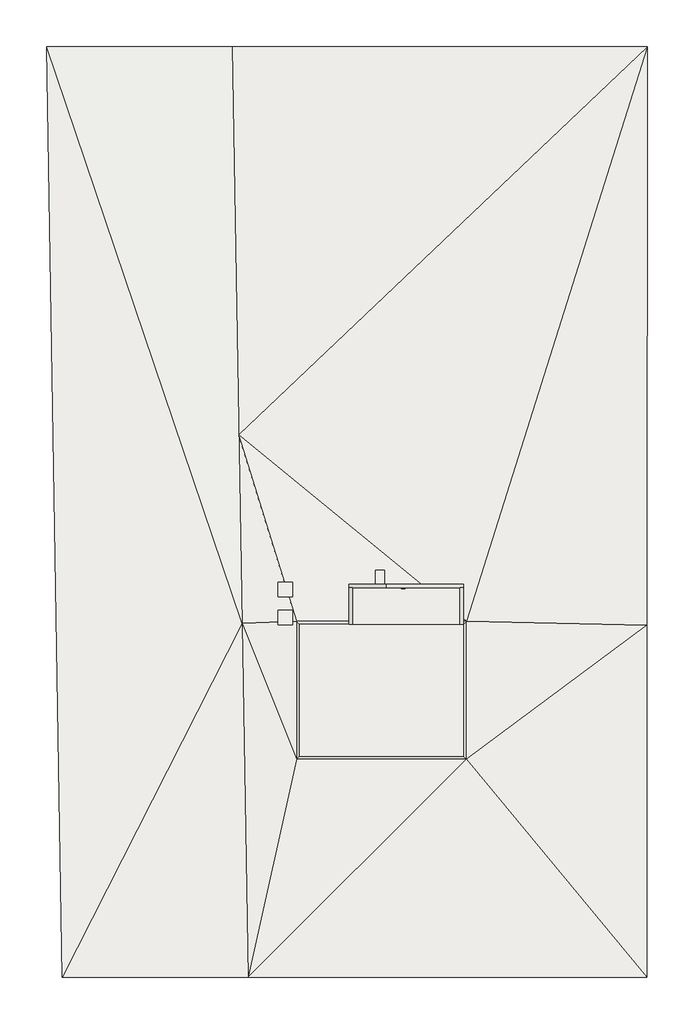
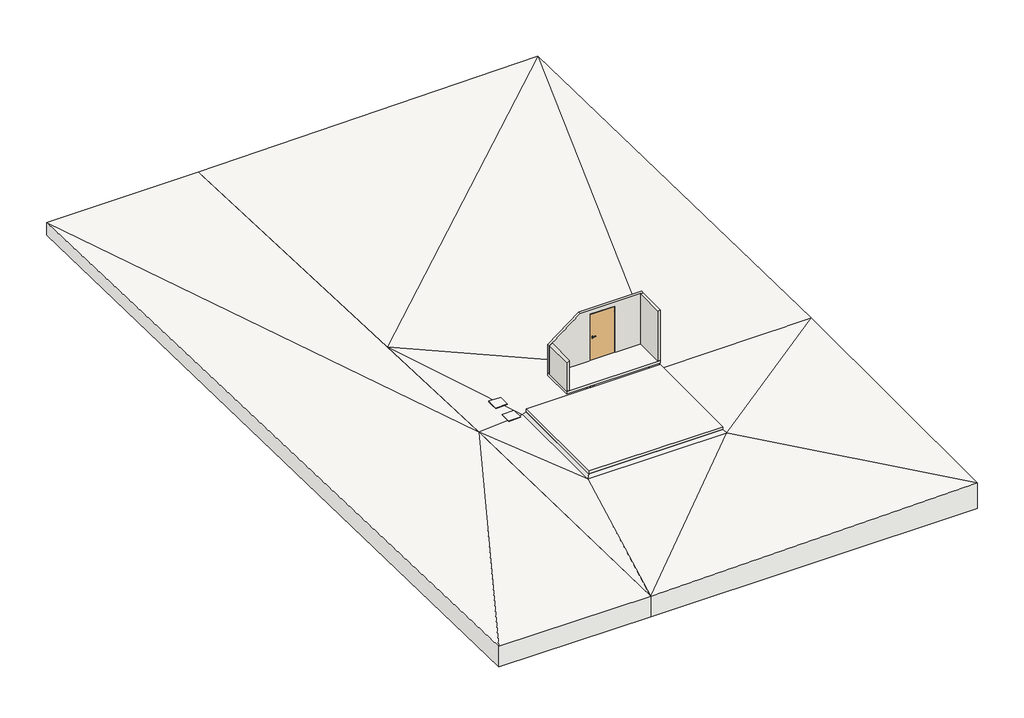
# Not in any storey: 7 slabs, 3 walls, 1 beam, 1 door.
"""IFC4 building model written with IfcOpenShell, lengths in millimetres."""

import ifcopenshell
import ifcopenshell.guid

model = None  # the IFC model being written
_history = None  # IfcOwnerHistory: only IFC2X3 demands one
_inside = {}  # id of a spatial element -> (the spatial element, [elements in it])
_under = {}  # id of a project, library or spatial element -> (it, [spatial elements below it])
_declared = {}  # id of a project -> (the project, [libraries it declares])
_typed = {}  # id of a type object -> (the type object, [elements of that type])
_made_of = {}  # id of a material, layer set ... -> (it, [elements and type objects made of it])


def new_model(schema):
    """Start an empty IFC model of exactly this schema.

    Asked for "IFC4X3", IfcOpenShell would pick the latest addendum, in which some entities
    have other attributes; the version numbers below select the first issue.
    IFC2X3 requires an IfcOwnerHistory on every rooted entity: one is made here for all.
    """
    global model, _history
    if schema == "IFC4X3":
        model = ifcopenshell.file(schema_version=(4, 3, 0, 0))
    else:
        model = ifcopenshell.file(schema=schema)
    _inside.clear()
    _under.clear()
    _declared.clear()
    _typed.clear()
    _made_of.clear()
    _history = None
    if model.schema == "IFC2X3":
        org = make("IfcOrganization", Name="unknown")
        user = make(
            "IfcPersonAndOrganization",
            ThePerson=make("IfcPerson", FamilyName="unknown"),
            TheOrganization=org,
        )
        app = make(
            "IfcApplication",
            ApplicationDeveloper=org,
            Version="unknown",
            ApplicationFullName="unknown",
            ApplicationIdentifier="unknown",
        )
        _history = make(
            "IfcOwnerHistory",
            OwningUser=user,
            OwningApplication=app,
            ChangeAction="ADDED",
            CreationDate=0,
        )
    return model


def make(cls, **values):
    """One entity of the class cls with the attributes given. An attribute that is None is left unset."""
    return model.create_entity(
        cls, **{name: value for name, value in values.items() if value is not None}
    )


def rooted(cls, **values):
    """An entity with a GlobalId (a new one), such as an element, a storey or a relation."""
    return make(cls, GlobalId=ifcopenshell.guid.new(), OwnerHistory=_history, **values)


def si_unit(unit_type, name, prefix=None):
    """IfcSIUnit, for example si_unit("LENGTHUNIT", "METRE", prefix="MILLI")."""
    return make("IfcSIUnit", UnitType=unit_type, Prefix=prefix, Name=name)


def assignment(units):
    """IfcUnitAssignment: the units of a project."""
    return None if units is None else make("IfcUnitAssignment", Units=units)


def point(xyz):
    """IfcCartesianPoint."""
    return None if xyz is None else make("IfcCartesianPoint", Coordinates=xyz)


def direction(xyz):
    """IfcDirection."""
    return None if xyz is None else make("IfcDirection", DirectionRatios=xyz)


def frame(location, z_axis=None, x_axis=None):
    """IfcAxis2Placement3D, a coordinate frame: its origin and axes. An axis left out is left unset."""
    return make(
        "IfcAxis2Placement3D",
        Location=point(location),
        Axis=direction(z_axis),
        RefDirection=direction(x_axis),
    )


def frame_2d(location, x_axis=None):
    """IfcAxis2Placement2D, a coordinate frame in the plane: its origin and x axis."""
    return make(
        "IfcAxis2Placement2D", Location=point(location), RefDirection=direction(x_axis)
    )


def origin():
    """The frame at (0, 0, 0) with its axes left unset."""
    return frame((0.0, 0.0, 0.0))


def place(relative_to, where):
    """IfcLocalPlacement: puts the frame where relative to a parent placement (None: the world)."""
    return make(
        "IfcLocalPlacement", PlacementRelTo=relative_to, RelativePlacement=where
    )


def context(
    kind, dimensions, precision=None, world=None, true_north=None, identifier=None
):
    """IfcGeometricRepresentationContext, for example the 3D "Model" context."""
    return make(
        "IfcGeometricRepresentationContext",
        ContextIdentifier=identifier,
        ContextType=kind,
        CoordinateSpaceDimension=dimensions,
        Precision=precision,
        WorldCoordinateSystem=world,
        TrueNorth=true_north,
    )


def project(units=None, contexts=None):
    """IfcProject with its units and contexts."""
    return rooted(
        "IfcProject",
        Name="project",
        RepresentationContexts=contexts,
        UnitsInContext=assignment(units),
    )


def spatial(cls, under=None, at=None, **own):
    """A site, building, storey or space (cls), placed at a placement, below another one or the project."""
    s = rooted(cls, ObjectPlacement=at, **own)
    if under is not None:
        _under.setdefault(under.id(), (under, []))[1].append(s)
    return s


def polyline(points):
    """IfcPolyline through the points."""
    return make("IfcPolyline", Points=[point(p) for p in points])


def circle_curve(where, radius):
    """IfcCircle in the frame where."""
    return make("IfcCircle", Position=where, Radius=radius)


def ellipse_curve(where, semi_axis1, semi_axis2):
    """IfcEllipse in the frame where."""
    return make(
        "IfcEllipse", Position=where, SemiAxis1=semi_axis1, SemiAxis2=semi_axis2
    )


def trimmed(basis, trim1, trim2, sense, master):
    """IfcTrimmedCurve: the piece of a basis curve between two trims."""
    return make(
        "IfcTrimmedCurve",
        BasisCurve=basis,
        Trim1=trim1,
        Trim2=trim2,
        SenseAgreement=sense,
        MasterRepresentation=master,
    )


def segment(curve, same_sense, transition):
    """IfcCompositeCurveSegment."""
    return make(
        "IfcCompositeCurveSegment",
        Transition=transition,
        SameSense=same_sense,
        ParentCurve=curve,
    )


def composite_curve(segments, self_intersect=None):
    """IfcCompositeCurve: segments joined end to end."""
    return make("IfcCompositeCurve", Segments=segments, SelfIntersect=self_intersect)


def outline(outer, holes=None, kind="AREA"):
    """IfcArbitraryClosedProfileDef: a profile drawn as a closed curve; with holes, ...WithVoids."""
    if holes is None:
        return make("IfcArbitraryClosedProfileDef", ProfileType=kind, OuterCurve=outer)
    return make(
        "IfcArbitraryProfileDefWithVoids",
        ProfileType=kind,
        OuterCurve=outer,
        InnerCurves=holes,
    )


def extrude(swept, where, along, depth):
    """IfcExtrudedAreaSolid: the profile swept, set in the frame where, extruded along a direction by depth."""
    return make(
        "IfcExtrudedAreaSolid",
        SweptArea=swept,
        Position=where,
        ExtrudedDirection=direction(along),
        Depth=depth,
    )


def faces_of(points, faces, orient=None, outer=None):
    """IfcFace entities. A face is a list of loops; a loop is a list of indices into points, from 0.

    orient and outer hold one flag for each loop. By default every Orientation is true, the
    first loop of a face is its IfcFaceOuterBound and the others are IfcFaceBound.
    """
    made = []
    for i, loops in enumerate(faces):
        bounds = []
        for j, loop in enumerate(loops):
            is_outer = j == 0 if outer is None else outer[i][j]
            bounds.append(
                make(
                    "IfcFaceOuterBound" if is_outer else "IfcFaceBound",
                    Bound=make("IfcPolyLoop", Polygon=[points[k] for k in loop]),
                    Orientation=True if orient is None else orient[i][j],
                )
            )
        made.append(make("IfcFace", Bounds=bounds))
    return made


def faceted_brep(points, faces, orient=None, outer=None, voids=None):
    """IfcFacetedBrep: a solid bounded by flat faces; with voids (closed shells), ...WithVoids."""
    shared = [point(p) for p in points]
    hull = make("IfcClosedShell", CfsFaces=faces_of(shared, faces, orient, outer))
    if voids is None:
        return make("IfcFacetedBrep", Outer=hull)
    return make(
        "IfcFacetedBrepWithVoids",
        Outer=hull,
        Voids=[
            make(cls, CfsFaces=faces_of(shared, fs, o, b)) for cls, fs, o, b in voids
        ],
    )


def shape(context_of_items, identifier, shape_type, items):
    """IfcShapeRepresentation: the items that make up one representation, for example the "Body"."""
    return make(
        "IfcShapeRepresentation",
        ContextOfItems=context_of_items,
        RepresentationIdentifier=identifier,
        RepresentationType=shape_type,
        Items=items,
    )


def source(mapping_origin, context_of_items, identifier, shape_type, items):
    """IfcRepresentationMap: a shape defined once, which mapped items show again and again."""
    return make(
        "IfcRepresentationMap",
        MappingOrigin=mapping_origin,
        MappedRepresentation=shape(context_of_items, identifier, shape_type, items),
    )


def transform(
    local_origin,
    x_axis=None,
    y_axis=None,
    z_axis=None,
    scale=None,
    scale2=None,
    scale3=None,
    uniform=True,
):
    """IfcCartesianTransformationOperator3D, or its non-uniform kind. x_axis, y_axis, z_axis: its Axis1, 2, 3."""
    if uniform:
        return make(
            "IfcCartesianTransformationOperator3D",
            Axis1=direction(x_axis),
            Axis2=direction(y_axis),
            LocalOrigin=point(local_origin),
            Scale=scale,
            Axis3=direction(z_axis),
        )
    return make(
        "IfcCartesianTransformationOperator3DnonUniform",
        Axis1=direction(x_axis),
        Axis2=direction(y_axis),
        LocalOrigin=point(local_origin),
        Scale=scale,
        Axis3=direction(z_axis),
        Scale2=scale2,
        Scale3=scale3,
    )


def mapped(mapping_source, mapping_target):
    """IfcMappedItem: shows the shape of a source again, moved by a transform."""
    return make(
        "IfcMappedItem", MappingSource=mapping_source, MappingTarget=mapping_target
    )


def made_of(thing, what):
    """Note that an element or type object is made of a material, layer set ...; save() writes the relation."""
    if what is not None:
        _made_of.setdefault(what.id(), (what, []))[1].append(thing)
    return thing


def element(
    cls,
    number,
    at=None,
    inside=None,
    cuts=None,
    type_object=None,
    material=None,
    context=None,
    identifier="Body",
    shape_type=None,
    held_by="IfcProductDefinitionShape",
    body=None,
    shapes=None,
    **own,
):
    """One element of the class cls, such as IfcWall. Its Tag is "e" and its number.

    at: its placement. inside: the storey or other place that contains it. cuts: it is an
    opening in that element (IfcRelVoidsElement). A single representation is given by context,
    identifier, shape_type and body (its items); several are given by shapes. held_by: the class
    of the entity that holds the representations. save() writes the other relations.
    """
    e = rooted(cls, Tag="e%d" % number, ObjectPlacement=at, **own)
    if body is not None:
        shapes = [shape(context, identifier, shape_type, body)]
    if shapes is not None:
        e.Representation = make(held_by, Representations=shapes)
    if inside is not None:
        _inside.setdefault(inside.id(), (inside, []))[1].append(e)
    if cuts is not None:
        rooted(
            "IfcRelVoidsElement", RelatingBuildingElement=cuts, RelatedOpeningElement=e
        )
    if type_object is not None:
        _typed.setdefault(type_object.id(), (type_object, []))[1].append(e)
    return made_of(e, material)


def aggregate(whole, parts):
    """IfcRelAggregates: a whole, such as a stair, and the parts it consists of."""
    return rooted("IfcRelAggregates", RelatingObject=whole, RelatedObjects=parts)


def save(model, path):
    """Write the relations noted so far, then the file.

    IfcRelAggregates (storeys below a building ...), IfcRelContainedInSpatialStructure (elements
    in a storey), IfcRelDefinesByType, IfcRelAssociatesMaterial and IfcRelDeclares: one each for
    every whole, place, type object, material and project.
    """
    for whole, parts in _under.values():
        aggregate(whole, parts)
    for where, things in _inside.values():
        rooted(
            "IfcRelContainedInSpatialStructure",
            RelatedElements=things,
            RelatingStructure=where,
        )
    for kind, things in _typed.values():
        rooted("IfcRelDefinesByType", RelatedObjects=things, RelatingType=kind)
    for what, things in _made_of.values():
        rooted("IfcRelAssociatesMaterial", RelatedObjects=things, RelatingMaterial=what)
    for by, libraries in _declared.values():
        rooted("IfcRelDeclares", RelatingContext=by, RelatedDefinitions=libraries)
    model.write(path)


def plane_surface(at):
    """IfcPlane: the flat surface through the origin of the frame at, square to its z axis."""
    return make("IfcPlane", Position=at)


def cylinder_surface(at, radius):
    """IfcCylindricalSurface: all points at the distance radius from the z axis of the frame at."""
    return make("IfcCylindricalSurface", Position=at, Radius=radius)


def advanced_brep(points, edges, surfaces, faces):
    """IfcAdvancedBrep: a solid bounded by faces that lie on surfaces and meet in shared edges.

    An edge is (start, end): straight between two places in points (the first is 0);
    or (start, end, curve); or (start, end, curve, False) where it runs against its curve.
    A face is (place in surfaces, loops), or (place, loops, False) where it looks against
    its surface's normal. A loop lists edges by number (the first is 1), with a minus sign
    where the edge is run from its end to its start. The first loop is the outer one.
    """
    corners = [point(p) for p in points]
    vertices = [make("IfcVertexPoint", VertexGeometry=c) for c in corners]
    made = []
    for start, end, *more in edges:
        made.append(
            make(
                "IfcEdgeCurve",
                EdgeStart=vertices[start],
                EdgeEnd=vertices[end],
                EdgeGeometry=more[0] if more else make("IfcPolyline", Points=[corners[start], corners[end]]),
                SameSense=more[1] if len(more) > 1 else True,
            )
        )
    hull = []
    for where, loops, *sense in faces:
        bounds = []
        for j, loop in enumerate(loops):
            ring = [make("IfcOrientedEdge", EdgeElement=made[abs(k) - 1], Orientation=k > 0) for k in loop]
            bounds.append(
                make(
                    "IfcFaceOuterBound" if j == 0 else "IfcFaceBound",
                    Bound=make("IfcEdgeLoop", EdgeList=ring),
                    Orientation=True,
                )
            )
        hull.append(make("IfcAdvancedFace", Bounds=bounds, FaceSurface=surfaces[where], SameSense=sense[0] if sense else True))
    return make("IfcAdvancedBrep", Outer=make("IfcClosedShell", CfsFaces=hull))


def holz_90_x_100_50d95c69(model_context):
    return source(origin(), model_context, "Body", "SweptSolid", [
        extrude(outline(polyline([(-638.5, -45.0), (-638.5, 45.0), (638.5, 45.0), (638.5, -45.0), (-638.5, -45.0)])), frame((0.0, 0.0, -50.0), z_axis=(0.0, 0.0, 1.0), x_axis=(1.0, 0.0, 0.0)), (0.0, 0.0, 1.0), 100.0),
    ])


def ml_1080_x_2101_9ecaf8c8(model_context):
    return source(origin(), model_context, "Body", "SolidModel", [
        faceted_brep([(515.0, -44.5, 0.0), (-515.0, -44.5, 0.0), (-515.0, -27.5, 0.0), (-500.0, -27.5, 0.0), (-500.0, 0.5, 0.0), (500.0, 0.5, 0.0), (500.0, -27.5, 0.0), (515.0, -27.5, 0.0), (515.0, -44.5, 2075.0), (-515.0, -44.5, 2075.0), (-515.0, -27.5, 2075.0), (-500.0, -27.5, 2060.0), (515.0, -27.5, 2075.0), (500.0, -27.5, 2060.0), (-500.0, 0.5, 2060.0), (500.0, 0.5, 2060.0)], [[[0, 1, 2, 3, 4, 5, 6, 7]], [[8, 9, 1, 0]], [[1, 9, 10, 2]], [[11, 3, 2, 10, 12, 7, 6, 13]], [[3, 11, 14, 4]], [[5, 4, 14, 15]], [[13, 6, 5, 15]], [[8, 0, 7, 12]], [[9, 8, 12, 10]], [[11, 13, 15, 14]]]),
        extrude(outline(composite_curve([segment(trimmed(circle_curve(frame_2d((527.0, -37.5)), 10.0), [point((517.0, -37.5))], [point((537.0, -37.5))], False, "CARTESIAN"), True, "CONTINUOUS"), segment(trimmed(circle_curve(frame_2d((527.0, -37.5)), 10.0), [point((537.0, -37.5))], [point((517.0, -37.5))], False, "CARTESIAN"), True, "CONTINUOUS")], self_intersect=False)), frame((0.0, 0.0, 1844.0), z_axis=(0.0, 0.0, 1.0), x_axis=(1.0, 0.0, 0.0)), (0.0, 0.0, 1.0), 25.0),
        extrude(outline(composite_curve([segment(trimmed(circle_curve(frame_2d((527.0, -37.5)), 10.0), [point((527.0, -27.5))], [point((518.339746, -32.5))], False, "CARTESIAN"), True, "CONTINUOUS"), segment(polyline([(518.339746, -32.5), (515.0, -32.5), (515.0, -27.5), (527.0, -27.5)]), True, "CONTINUOUS")], self_intersect=False)), frame((0.0, 0.0, 1794.0), z_axis=(0.0, 0.0, 1.0), x_axis=(1.0, 0.0, 0.0)), (0.0, 0.0, 1.0), 50.0),
        extrude(outline(composite_curve([segment(trimmed(circle_curve(frame_2d((527.0, -37.5)), 10.0), [point((517.0, -37.5))], [point((537.0, -37.5))], False, "CARTESIAN"), True, "CONTINUOUS"), segment(trimmed(circle_curve(frame_2d((527.0, -37.5)), 10.0), [point((537.0, -37.5))], [point((517.0, -37.5))], False, "CARTESIAN"), True, "CONTINUOUS")], self_intersect=False)), frame((0.0, 0.0, 1769.0), z_axis=(0.0, 0.0, 1.0), x_axis=(1.0, 0.0, 0.0)), (0.0, 0.0, 1.0), 25.0),
        extrude(outline(composite_curve([segment(trimmed(circle_curve(frame_2d((527.0, -37.5)), 10.0), [point((517.0, -37.5))], [point((537.0, -37.5))], False, "CARTESIAN"), True, "CONTINUOUS"), segment(trimmed(circle_curve(frame_2d((527.0, -37.5)), 10.0), [point((537.0, -37.5))], [point((517.0, -37.5))], False, "CARTESIAN"), True, "CONTINUOUS")], self_intersect=False)), frame((0.0, 0.0, 266.0), z_axis=(0.0, 0.0, 1.0), x_axis=(1.0, 0.0, 0.0)), (0.0, 0.0, 1.0), 25.0),
        extrude(outline(composite_curve([segment(trimmed(circle_curve(frame_2d((527.0, -37.5)), 10.0), [point((527.0, -27.5))], [point((518.339746, -32.5))], False, "CARTESIAN"), True, "CONTINUOUS"), segment(polyline([(518.339746, -32.5), (515.0, -32.5), (515.0, -27.5), (527.0, -27.5)]), True, "CONTINUOUS")], self_intersect=False)), frame((0.0, 0.0, 216.0), z_axis=(0.0, 0.0, 1.0), x_axis=(1.0, 0.0, 0.0)), (0.0, 0.0, 1.0), 50.0),
        extrude(outline(composite_curve([segment(trimmed(circle_curve(frame_2d((527.0, -37.5)), 10.0), [point((517.0, -37.5))], [point((537.0, -37.5))], False, "CARTESIAN"), True, "CONTINUOUS"), segment(trimmed(circle_curve(frame_2d((527.0, -37.5)), 10.0), [point((537.0, -37.5))], [point((517.0, -37.5))], False, "CARTESIAN"), True, "CONTINUOUS")], self_intersect=False)), frame((0.0, 0.0, 191.0), z_axis=(0.0, 0.0, 1.0), x_axis=(1.0, 0.0, 0.0)), (0.0, 0.0, 1.0), 25.0),
        advanced_brep(
        [(-420.0, -54.5, 1050.0), (-440.0, -54.5, 1050.0), (-440.0, -104.5, 1050.0), (-420.0, -84.5, 1050.0), (-310.0, -84.5, 1050.0), (-310.0, -104.5, 1050.0)],
        [
            (0, 1, circle_curve(frame((-430.0, -54.5, 1050.0), z_axis=(0.0, 1.0, 0.0), x_axis=(-1.0, 0.0, 0.0)), 10.0)),
            (1, 0, circle_curve(frame((-430.0, -54.5, 1050.0), z_axis=(0.0, 1.0, 0.0), x_axis=(-1.0, 0.0, 0.0)), 10.0)),
            (1, 2),
            (2, 3, ellipse_curve(frame((-430.0, -94.5, 1050.0), z_axis=(-0.7071067811865531, 0.7071067811865419, 0.0), x_axis=(0.707106781186542, 0.707106781186553, 0.0)), 14.1421356, 10.0)),
            (3, 0),
            (3, 2, ellipse_curve(frame((-430.0, -94.5, 1050.0), z_axis=(-0.7071067811865531, 0.7071067811865419, 0.0), x_axis=(0.707106781186542, 0.707106781186553, 0.0)), 14.1421356, 10.0)),
            (4, 5, circle_curve(frame((-310.0, -94.5, 1050.0), z_axis=(1.0, 0.0, 0.0), x_axis=(0.0, -1.0, 0.0)), 10.0)),
            (5, 4, circle_curve(frame((-310.0, -94.5, 1050.0), z_axis=(1.0, 0.0, 0.0), x_axis=(0.0, -1.0, 0.0)), 10.0)),
            (2, 5),
            (4, 3),
        ],
        [
            plane_surface(frame((-430.0, -54.5, 1050.0), z_axis=(0.0, 1.0, 0.0), x_axis=(0.0, 0.0, 1.0))),
            cylinder_surface(frame((-430.0, -54.5, 1050.0), z_axis=(0.0, 1.0, 0.0), x_axis=(-1.0, 0.0, 0.0)), 10.0),
            plane_surface(frame((-310.0, -94.5, 1050.0), z_axis=(1.0, 0.0, 0.0), x_axis=(0.0, 0.0, 1.0))),
            cylinder_surface(frame((-430.0, -94.5, 1050.0), z_axis=(-1.0, 0.0, 0.0), x_axis=(0.0, -1.0, 0.0)), 10.0),
        ],
        [
            (0, [[1, 2]]),
            (1, [[3, 4, 5, -2]]),
            (1, [[-5, 6, -3, -1]]),
            (2, [[7, 8]]),
            (3, [[9, -7, 10, -4]]),
            (3, [[-10, -8, -9, -6]]),
        ],
    ),
        extrude(outline(composite_curve([segment(trimmed(circle_curve(frame_2d((990.0, -430.0)), 20.0), [point((990.0, -450.0))], [point((990.0, -410.0))], False, "CARTESIAN"), True, "CONTINUOUS"), segment(trimmed(circle_curve(frame_2d((990.0, -430.0)), 20.0), [point((990.0, -410.0))], [point((990.0, -450.0))], False, "CARTESIAN"), True, "CONTINUOUS")], self_intersect=False), holes=[composite_curve([segment(polyline([(976.4601385, -432.397268), (988.4749012, -432.397268)]), True, "CONTINUOUS"), segment(trimmed(circle_curve(frame_2d((995.0361633, -430.0)), 6.9854888), [point((988.4749012, -432.397268))], [point((988.4749012, -427.602732))], True, "CARTESIAN"), True, "CONTINUOUS"), segment(polyline([(988.4749012, -427.602732), (976.4601385, -427.602732)]), True, "CONTINUOUS"), segment(trimmed(circle_curve(frame_2d((976.4601385, -430.0)), 2.397268), [point((976.4601385, -427.602732))], [point((976.4601385, -432.397268))], True, "CARTESIAN"), True, "CONTINUOUS")], self_intersect=False)]), frame((0.0, -54.5, 0.0), z_axis=(0.0, 1.0, 0.0), x_axis=(0.0, 0.0, 1.0)), (0.0, 0.0, 1.0), 10.0),
        advanced_brep(
        [(-420.0, -54.5, 1050.0), (-440.0, -54.5, 1050.0), (-440.0, -104.5, 1050.0), (-420.0, -84.5, 1050.0), (-310.0, -84.5, 1050.0), (-310.0, -104.5, 1050.0)],
        [
            (0, 1, circle_curve(frame((-430.0, -54.5, 1050.0), z_axis=(0.0, 1.0, 0.0), x_axis=(-1.0, 0.0, 0.0)), 10.0)),
            (1, 0, circle_curve(frame((-430.0, -54.5, 1050.0), z_axis=(0.0, 1.0, 0.0), x_axis=(-1.0, 0.0, 0.0)), 10.0)),
            (1, 2),
            (2, 3, ellipse_curve(frame((-430.0, -94.5, 1050.0), z_axis=(-0.7071067811865537, 0.7071067811865414, 0.0), x_axis=(0.7071067811865414, 0.7071067811865536, 0.0)), 14.1421356, 10.0)),
            (3, 0),
            (3, 2, ellipse_curve(frame((-430.0, -94.5, 1050.0), z_axis=(-0.7071067811865537, 0.7071067811865414, 0.0), x_axis=(0.7071067811865414, 0.7071067811865536, 0.0)), 14.1421356, 10.0)),
            (4, 5, circle_curve(frame((-310.0, -94.5, 1050.0), z_axis=(1.0, 0.0, 0.0), x_axis=(0.0, -1.0, 0.0)), 10.0)),
            (5, 4, circle_curve(frame((-310.0, -94.5, 1050.0), z_axis=(1.0, 0.0, 0.0), x_axis=(0.0, -1.0, 0.0)), 10.0)),
            (2, 5),
            (4, 3),
        ],
        [
            plane_surface(frame((-430.0, -54.5, 1050.0), z_axis=(0.0, 1.0, 0.0), x_axis=(0.0, 0.0, 1.0))),
            cylinder_surface(frame((-430.0, -54.5, 1050.0), z_axis=(0.0, 1.0, 0.0), x_axis=(-1.0, 0.0, 0.0)), 10.0),
            plane_surface(frame((-310.0, -94.5, 1050.0), z_axis=(1.0, 0.0, 0.0), x_axis=(0.0, 0.0, 1.0))),
            cylinder_surface(frame((-430.0, -94.5, 1050.0), z_axis=(-1.0, 0.0, 0.0), x_axis=(0.0, -1.0, 0.0)), 10.0),
        ],
        [
            (0, [[1, 2]]),
            (1, [[3, 4, 5, -2]]),
            (1, [[-5, 6, -3, -1]]),
            (2, [[7, 8]]),
            (3, [[9, -7, 10, -4]]),
            (3, [[-10, -8, -9, -6]]),
        ],
    ),
        extrude(outline(composite_curve([segment(trimmed(circle_curve(frame_2d((1050.0, -430.0)), 20.0), [point((1050.0, -450.0))], [point((1050.0, -410.0))], False, "CARTESIAN"), True, "CONTINUOUS"), segment(trimmed(circle_curve(frame_2d((1050.0, -430.0)), 20.0), [point((1050.0, -410.0))], [point((1050.0, -450.0))], False, "CARTESIAN"), True, "CONTINUOUS")], self_intersect=False)), frame((0.0, -54.5, 0.0), z_axis=(0.0, 1.0, 0.0), x_axis=(0.0, 0.0, 1.0)), (0.0, 0.0, 1.0), 10.0),
        advanced_brep(
        [(-420.0, 10.5, 1050.0), (-440.0, 10.5, 1050.0), (-420.0, 40.5, 1050.0), (-440.0, 60.5, 1050.0), (-310.0, 40.5, 1050.0), (-310.0, 60.5, 1050.0)],
        [
            (0, 1, circle_curve(frame((-430.0, 10.5, 1050.0), z_axis=(0.0, -1.0, 0.0), x_axis=(-1.0, 0.0, 0.0)), 10.0)),
            (1, 0, circle_curve(frame((-430.0, 10.5, 1050.0), z_axis=(0.0, -1.0, 0.0), x_axis=(-1.0, 0.0, 0.0)), 10.0)),
            (0, 2),
            (2, 3, ellipse_curve(frame((-430.0, 50.5, 1050.0), z_axis=(-0.7071067811865486, -0.7071067811865464, 0.0), x_axis=(0.7071067811865464, -0.7071067811865488, 0.0)), 14.1421356, 10.0)),
            (3, 1),
            (3, 2, ellipse_curve(frame((-430.0, 50.5, 1050.0), z_axis=(-0.7071067811865486, -0.7071067811865464, 0.0), x_axis=(0.7071067811865464, -0.7071067811865488, 0.0)), 14.1421356, 10.0)),
            (4, 5, circle_curve(frame((-310.0, 50.5, 1050.0), z_axis=(1.0, 0.0, 0.0), x_axis=(0.0, 1.0, 0.0)), 10.0)),
            (5, 4, circle_curve(frame((-310.0, 50.5, 1050.0), z_axis=(1.0, 0.0, 0.0), x_axis=(0.0, 1.0, 0.0)), 10.0)),
            (2, 4),
            (5, 3),
        ],
        [
            plane_surface(frame((-430.0, 10.5, 1050.0), z_axis=(0.0, -1.0, 0.0), x_axis=(0.0, 0.0, 1.0))),
            cylinder_surface(frame((-430.0, 10.5, 1050.0), z_axis=(0.0, -1.0, 0.0), x_axis=(-1.0, 0.0, 0.0)), 10.0),
            plane_surface(frame((-310.0, 50.5, 1050.0), z_axis=(1.0, 0.0, 0.0), x_axis=(0.0, 0.0, 1.0))),
            cylinder_surface(frame((-430.0, 50.5, 1050.0), z_axis=(-1.0, 0.0, 0.0), x_axis=(0.0, 1.0, 0.0)), 10.0),
        ],
        [
            (0, [[1, 2]]),
            (1, [[-1, 3, 4, 5]]),
            (1, [[-2, -5, 6, -3]]),
            (2, [[7, 8]]),
            (3, [[-4, 9, -8, 10]]),
            (3, [[-6, -10, -7, -9]]),
        ],
    ),
        extrude(outline(composite_curve([segment(trimmed(circle_curve(frame_2d((990.0, -430.0)), 20.0), [point((990.0, -450.0))], [point((990.0, -410.0))], False, "CARTESIAN"), True, "CONTINUOUS"), segment(trimmed(circle_curve(frame_2d((990.0, -430.0)), 20.0), [point((990.0, -410.0))], [point((990.0, -450.0))], False, "CARTESIAN"), True, "CONTINUOUS")], self_intersect=False), holes=[composite_curve([segment(polyline([(976.4601385, -432.397268), (988.4749012, -432.397268)]), True, "CONTINUOUS"), segment(trimmed(circle_curve(frame_2d((995.0361633, -430.0)), 6.9854888), [point((988.4749012, -432.397268))], [point((988.4749012, -427.602732))], True, "CARTESIAN"), True, "CONTINUOUS"), segment(polyline([(988.4749012, -427.602732), (976.4601385, -427.602732)]), True, "CONTINUOUS"), segment(trimmed(circle_curve(frame_2d((976.4601385, -430.0)), 2.397268), [point((976.4601385, -427.602732))], [point((976.4601385, -432.397268))], True, "CARTESIAN"), True, "CONTINUOUS")], self_intersect=False)]), frame((0.0, 0.5, 0.0), z_axis=(0.0, 1.0, 0.0), x_axis=(0.0, 0.0, 1.0)), (0.0, 0.0, 1.0), 10.0),
        advanced_brep(
        [(-420.0, 10.5, 1050.0), (-440.0, 10.5, 1050.0), (-420.0, 40.5, 1050.0), (-440.0, 60.5, 1050.0), (-310.0, 40.5, 1050.0), (-310.0, 60.5, 1050.0)],
        [
            (0, 1, circle_curve(frame((-430.0, 10.5, 1050.0), z_axis=(0.0, -1.0, 0.0), x_axis=(-1.0, 0.0, 0.0)), 10.0)),
            (1, 0, circle_curve(frame((-430.0, 10.5, 1050.0), z_axis=(0.0, -1.0, 0.0), x_axis=(-1.0, 0.0, 0.0)), 10.0)),
            (0, 2),
            (2, 3, ellipse_curve(frame((-430.0, 50.5, 1050.0), z_axis=(-0.7071067811865491, -0.7071067811865459, 0.0), x_axis=(0.7071067811865458, -0.7071067811865492, 0.0)), 14.1421356, 10.0)),
            (3, 1),
            (3, 2, ellipse_curve(frame((-430.0, 50.5, 1050.0), z_axis=(-0.7071067811865491, -0.7071067811865459, 0.0), x_axis=(0.7071067811865458, -0.7071067811865492, 0.0)), 14.1421356, 10.0)),
            (4, 5, circle_curve(frame((-310.0, 50.5, 1050.0), z_axis=(1.0, 0.0, 0.0), x_axis=(0.0, 1.0, 0.0)), 10.0)),
            (5, 4, circle_curve(frame((-310.0, 50.5, 1050.0), z_axis=(1.0, 0.0, 0.0), x_axis=(0.0, 1.0, 0.0)), 10.0)),
            (2, 4),
            (5, 3),
        ],
        [
            plane_surface(frame((-430.0, 10.5, 1050.0), z_axis=(0.0, -1.0, 0.0), x_axis=(0.0, 0.0, 1.0))),
            cylinder_surface(frame((-430.0, 10.5, 1050.0), z_axis=(0.0, -1.0, 0.0), x_axis=(-1.0, 0.0, 0.0)), 10.0),
            plane_surface(frame((-310.0, 50.5, 1050.0), z_axis=(1.0, 0.0, 0.0), x_axis=(0.0, 0.0, 1.0))),
            cylinder_surface(frame((-430.0, 50.5, 1050.0), z_axis=(-1.0, 0.0, 0.0), x_axis=(0.0, 1.0, 0.0)), 10.0),
        ],
        [
            (0, [[1, 2]]),
            (1, [[-1, 3, 4, 5]]),
            (1, [[-2, -5, 6, -3]]),
            (2, [[7, 8]]),
            (3, [[-4, 9, -8, 10]]),
            (3, [[-6, -10, -7, -9]]),
        ],
    ),
        extrude(outline(composite_curve([segment(trimmed(circle_curve(frame_2d((1050.0, -430.0)), 20.0), [point((1050.0, -450.0))], [point((1050.0, -410.0))], False, "CARTESIAN"), True, "CONTINUOUS"), segment(trimmed(circle_curve(frame_2d((1050.0, -430.0)), 20.0), [point((1050.0, -410.0))], [point((1050.0, -450.0))], False, "CARTESIAN"), True, "CONTINUOUS")], self_intersect=False)), frame((0.0, 0.5, 0.0), z_axis=(0.0, 1.0, 0.0), x_axis=(0.0, 0.0, 1.0)), (0.0, 0.0, 1.0), 10.0),
        faceted_brep([(-500.0, -27.5, 0.0), (-540.0, -27.5, 0.0), (-540.0, 27.5, 0.0), (-485.0, 27.5, 0.0), (-485.0, 0.5, 0.0), (-500.0, 0.5, 0.0), (-500.0, 0.5, 2060.0), (-500.0, -27.5, 2060.0), (-485.0, 0.5, 2045.0), (485.0, 0.5, 2045.0), (485.0, 0.5, 0.0), (500.0, 0.5, 0.0), (500.0, 0.5, 2060.0), (-485.0, 27.5, 2045.0), (-540.0, 27.5, 2100.0), (540.0, 27.5, 2100.0), (540.0, 27.5, 0.0), (485.0, 27.5, 0.0), (485.0, 27.5, 2045.0), (-540.0, -27.5, 2100.0), (500.0, -27.5, 2060.0), (500.0, -27.5, 0.0), (540.0, -27.5, 0.0), (540.0, -27.5, 2100.0)], [[[0, 1, 2, 3, 4, 5]], [[5, 6, 7, 0]], [[4, 8, 9, 10, 11, 12, 6, 5]], [[3, 13, 8, 4]], [[2, 14, 15, 16, 17, 18, 13, 3]], [[1, 19, 14, 2]], [[0, 7, 20, 21, 22, 23, 19, 1]], [[23, 22, 16, 15]], [[21, 11, 10, 17, 16, 22]], [[12, 11, 21, 20]], [[18, 17, 10, 9]], [[19, 23, 15, 14]], [[13, 18, 9, 8]], [[6, 12, 20, 7]]]),
    ])


def einzelfundament_stb_500_x_500_x_300_3619195b(model_context):
    return source(origin(), model_context, "Body", "SweptSolid", [
        extrude(outline(polyline([(250.0, 250.0), (250.0, -250.0), (-250.0, -250.0), (-250.0, 250.0), (250.0, 250.0)])), frame((0.0, 0.0, -300.0), z_axis=(0.0, 0.0, 1.0), x_axis=(1.0, 0.0, 0.0)), (0.0, 0.0, 1.0), 300.0),
    ])


model = new_model("IFC4")

# Units and contexts
model_context = context("Model", 3, world=origin())
ifc_project = project(units=[si_unit("LENGTHUNIT", "METRE", prefix="MILLI")], contexts=[model_context])

# Site, building
site = spatial("IfcSite", under=ifc_project)
building = spatial("IfcBuilding", under=site)

# Beam
placement = place(None, origin())
holz_90_x_100_shape = holz_90_x_100_50d95c69(model_context)
element("IfcBeam", 1, ObjectType="Holz Träger - rechteckig : Holz 90 x 100", at=placement, inside=building, context=model_context, shape_type="MappedRepresentation", body=[
    mapped(holz_90_x_100_shape, transform((9139.843584, 9402.7803922, -270.0), x_axis=(0.0, -1.0, 0.0), y_axis=(1.0, 0.0, 0.0), z_axis=(0.0, 0.0, 1.0))),
])

# Door
ml_1080_x_2101_shape = ml_1080_x_2101_9ecaf8c8(model_context)
element("IfcDoor", 2, ObjectType="TU DF 1 - Pfostenstock Falztüre : ML - 1080 x 2101", at=placement, inside=building, context=model_context, shape_type="MappedRepresentation", body=[
    mapped(ml_1080_x_2101_shape, transform((10322.9226469, 10084.5272422, -100.0), x_axis=(1.0, 0.0, 0.0), y_axis=(0.0, 1.0, 0.0), z_axis=(0.0, 0.0, 1.0))),
])

# Slabs
element("IfcSlab", 3, ObjectType="WD 120 hart", at=placement, inside=building, context=model_context, shape_type="SweptSolid", body=[
    extrude(outline(polyline([(12052.9226469, 8754.5272422), (12052.9226469, 4144.5272422), (6332.9226469, 4144.5272422), (6332.9226469, 8754.5272422), (12052.9226469, 8754.5272422)])), frame((0.0, 0.0, -420.0), z_axis=(0.0, 0.0, 1.0), x_axis=(1.0, 0.0, 0.0)), (0.0, 0.0, 1.0), 120.0),
])
element("IfcSlab", 4, ObjectType="AL Grünfläche", at=placement, inside=building, context=model_context, shape_type="Brep", body=[
    faceted_brep([(18451.9869184, 28873.5069375, -1560.9044), (18448.9881934, 8708.0675618, -1560.9044), (18447.1199211, -3557.1970822, -1560.9044), (4539.8145475, -3555.0786825, -1560.9044), (4328.9058413, 8779.6808532, -1560.9044), (3985.3098426, 28871.3033595, -1560.9044), (18451.9869184, 28873.5069375, -838.5044), (18448.9881934, 8708.0675618, -398.9094998), (18447.1199211, -3557.1970822, -400.9044), (4539.8145475, -3555.0786825, -642.6582175), (4328.9058413, 8779.6808532, -645.3457), (4216.6527387, 15343.6249499, -761.8881193), (3985.3098426, 28871.3033595, -1002.0712139), (6232.9226469, 4044.5272422, -560.9044), (12152.9226469, 4044.5272422, -560.9044), (6332.9226469, 8754.5272422, -420.0), (6332.9226469, 4144.5272422, -420.0), (12052.9226469, 4144.5272422, -420.0), (12052.9226469, 8754.5272422, -420.0), (12152.9226469, 8854.5272422, -560.9044), (6232.9226469, 8854.5272422, -560.9044)], [[[0, 1, 2, 3, 4, 5]], [[1, 0, 6, 7]], [[2, 1, 7, 8]], [[3, 2, 8, 9]], [[4, 3, 9, 10]], [[5, 4, 10, 11, 12]], [[0, 5, 12, 6]], [[10, 9, 13]], [[9, 8, 14]], [[12, 11, 6]], [[8, 7, 14]], [[15, 16, 17, 18]], [[15, 18, 19, 20]], [[7, 19, 14]], [[9, 14, 13]], [[17, 14, 19, 18]], [[16, 13, 14, 17]], [[15, 20, 13, 16]], [[10, 20, 11]], [[10, 13, 20]], [[11, 20, 19]], [[11, 19, 6]], [[7, 6, 19]]]),
])
element("IfcSlab", 5, ObjectType="AL Asphalt", at=placement, inside=building, context=model_context, shape_type="Brep", body=[
    faceted_brep([(4328.9058413, 8779.6808532, -1560.9044), (4539.8145475, -3555.0786825, -1560.9044), (-1931.6832245, -3555.0786825, -1560.9044), (-2486.2197616, 28871.3033595, -1560.9044), (3985.3098426, 28871.3033595, -1560.9044), (4328.9058413, 8779.6808532, -645.3456973), (4539.8145475, -3555.0786825, -642.6582175), (-1931.6832245, -3555.0786825, -642.7044), (-2486.2197616, 28871.3033595, -1002.1044), (3985.3098426, 28871.3033595, -1002.0712139)], [[[0, 1, 2, 3, 4]], [[1, 0, 5, 6]], [[2, 1, 6, 7]], [[3, 2, 7, 8]], [[4, 3, 8, 9]], [[0, 4, 9, 5]], [[9, 8, 5]], [[8, 7, 5]], [[7, 6, 5]]]),
])
element("IfcSlab", 6, ObjectType="Einzelfundament : STB 1870 x 300 x 500", at=placement, inside=building, context=model_context, shape_type="SweptSolid", body=[
    extrude(outline(polyline([(8989.843584, 10634.0293422), (9289.843584, 10634.0293422), (9289.843584, 8764.0293422), (8989.843584, 8764.0293422), (8989.843584, 10634.0293422)])), frame((0.0, 0.0, -820.0), z_axis=(0.0, 0.0, 1.0), x_axis=(1.0, 0.0, 0.0)), (0.0, 0.0, 1.0), 500.0),
])
einzelfundament_stb_500_x_500_x_300_shape = einzelfundament_stb_500_x_500_x_300_3619195b(model_context)
element("IfcSlab", 7, ObjectType="Einzelfundament : STB 500 x 500 x 300", at=placement, inside=building, context=model_context, shape_type="MappedRepresentation", body=[
    mapped(einzelfundament_stb_500_x_500_x_300_shape, transform((5835.8451291, 8984.5272422, -560.9044), x_axis=(1.0, 0.0, 0.0), y_axis=(0.0, 1.0, 0.0), z_axis=(0.0, 0.0, 1.0))),
])
element("IfcSlab", 8, ObjectType="Einzelfundament : STB 500 x 500 x 300", at=placement, inside=building, context=model_context, shape_type="MappedRepresentation", body=[
    mapped(einzelfundament_stb_500_x_500_x_300_shape, transform((5835.8451291, 9958.5272422, -560.9044), x_axis=(1.0, 0.0, 0.0), y_axis=(0.0, 1.0, 0.0), z_axis=(0.0, 0.0, 1.0))),
])
element("IfcSlab", 9, ObjectType="KLH 120", at=placement, inside=building, context=model_context, shape_type="SweptSolid", body=[
    extrude(outline(polyline([(12052.9226469, 8754.5272422), (8052.9226469, 8754.5272422), (8052.9226469, 10144.5272422), (12052.9226469, 10144.5272422), (12052.9226469, 8754.5272422)])), frame((0.0, 0.0, -220.0), z_axis=(0.0, 0.0, 1.0), x_axis=(1.0, 0.0, 0.0)), (0.0, 0.0, 1.0), 120.0),
])

# Walls
element("IfcWall", 10, ObjectType="KLH 120", at=placement, inside=building, context=model_context, shape_type="Brep", body=[
    faceted_brep([(12052.9226469, 10144.5272422, 2170.0), (12052.9226469, 10144.5272422, -100.0), (10862.9226469, 10144.5272422, -100.0), (10862.9226469, 10144.5272422, 2000.0), (9782.9226469, 10144.5272422, 2000.0), (9782.9226469, 10144.5272422, -100.0), (8052.9226469, 10144.5272422, -100.0), (8052.9226469, 10144.5272422, 1165.8420612), (9374.1830316, 10144.5272422, 2170.0), (12052.9226469, 10024.5272422, -100.0), (12052.9226469, 10024.5272422, 2170.0), (11932.9226469, 10024.5272422, 2170.0), (9374.1830316, 10024.5272422, 2170.0), (8172.9226469, 10024.5272422, 1257.0420654), (8052.9226469, 10024.5272422, 1165.8420612), (8052.9226469, 10024.5272422, -100.0), (8172.9226469, 10024.5272422, -100.0), (9782.9226469, 10024.5272422, -100.0), (9782.9226469, 10024.5272422, 2000.0), (10862.9226469, 10024.5272422, 2000.0), (10862.9226469, 10024.5272422, -100.0), (11932.9226469, 10024.5272422, -100.0)], [[[0, 1, 2, 3, 4, 5, 6, 7, 8]], [[9, 10, 11, 12, 13, 14, 15, 16, 17, 18, 19, 20, 21]], [[1, 9, 21, 20, 2]], [[15, 6, 5, 17, 16]], [[19, 3, 2, 20]], [[4, 18, 17, 5]], [[3, 19, 18, 4]], [[1, 0, 10, 9]], [[7, 6, 15, 14]], [[10, 0, 8, 12, 11]], [[7, 14, 13, 12, 8]]]),
])
element("IfcWall", 11, ObjectType="KLH 120", at=placement, inside=building, context=model_context, shape_type="SweptSolid", body=[
    extrude(outline(polyline([(12052.9226469, 10024.5272422), (12052.9226469, 8754.5272422), (11932.9226469, 8754.5272422), (11932.9226469, 10024.5272422), (12052.9226469, 10024.5272422)])), frame((0.0, 0.0, -100.0), z_axis=(0.0, 0.0, 1.0), x_axis=(1.0, 0.0, 0.0)), (0.0, 0.0, 1.0), 2270.0),
])
element("IfcWall", 12, ObjectType="KLH 120", at=placement, inside=building, context=model_context, shape_type="SweptSolid", body=[
    extrude(outline(polyline([(-100.0, 8172.9226469), (1257.0420654, 8172.9226469), (1165.8420612, 8052.9226469), (-100.0, 8052.9226469), (-100.0, 8172.9226469)])), frame((0.0, 8754.5272422, 0.0), z_axis=(0.0, 1.0, 0.0), x_axis=(0.0, 0.0, 1.0)), (0.0, 0.0, 1.0), 1270.0),
])

save(model, "model.ifc")

# Revit data of these elements
# Type "Holz Träger - rechteckig : Holz 90 x 100"
#   Type Comments = "B/H=9/10cm"
#   Perimeter = 0.38 m²/m
#   Moment of Inertia strong axis = 750.00 cm⁴
#   Moment of Inertia weak axis = 607.50 cm⁴
#   Section Area = 90.0 cm²
#   Length [instance default] = 1.524 m
#   Height = 10.0 cm
#   Width = 9.0 cm
#   B = 0.090 m
#   H = 0.100 m
#   Structural Material = Holz - C 24 Cl.1
# Type "TU DF 1 - Pfostenstock Falztüre : ML - 1080 x 2101"
#   Type IfcGUID = "32vBIxahr8bQdQw1D1hUMo"
#   Type Mark = "235"
#   Operation = "SINGLE_SWING_RIGHT"
#   URL = "http://www.autodesk.de/BIM"
#   Type Comments = "Pfostenstock Falztüre"
#   Form Tür = "rechteckig"
#   Description = "1-teilig"
#   Ausführung Zarge = "Blockzarge"
#   Anzahl Seitenteile = "0"
#   Anzahl Oberlichter = "0"
#   Anzahl Flügel = "einflügelig"
#   Anschlag- / Bewegungsart Tür = "Drehflügeltür"
#   Analytic Construction = "<Keine Auswahl>"
#   Winkel Öffnungsbogen [instance default] = 90.00°
#   Wandstärke Gesamt [instance default] = 0.300 m
#   Wandstärke [instance default] = 0.300 m
#   Wandaufbau Gegenbandseite [instance default] = 0.000 m
#   Wandaufbau Bandseite [instance default] = 0.000 m
#   Rough Height [instance default] = 2.280 m
#   Rough Width = 1.080 m
#   Randabstand Öffnungssymbol = 0.000 m
#   Rahmentiefe = 0.055 m
#   Rahmendicke = 0.055 m
#   Höhe ab FBOK = 2.100 m
#   Fußbodenaufbau [instance default] = 0.180 m
#   Height [instance default] = 2.100 m
#   Falztiefe = 0.028 m
#   Falzaufschlag = 0.017 m
#   Einbautiefe [instance default] = 0.080 m
#   Durchgangshöhe = 2.045 m
#   Durchgangsbreite = 0.970 m
#   Drückerhöhe = 1.050 m
#   Thickness = 0.045 m
#   Width = 1.080 m
#   B_Einbautiefe [instance default] = 0.1225 m
#   Angabe Maueröffnungsmaß Höhe = 2.100 m
#   Angabe Maueröffnungsmaß Breite = 1.080 m
#   Angabe Lichter Durchgang Höhe = 2.000 m
#   Angabe Lichter Durchgang Breite = 0.800 m
#   Zylinderrosette [instance default] = yes
#   Tür mit Anschlag [instance default] = no
#   Pfostenstock Wandmittig eingebaut [instance default] = yes
#   Kollisionskörper einschalten [instance default] = no
#   Knauf Innenseite [instance default] = no
#   Knauf Außenseite [instance default] = no
#   Höhe ab FBOK berechnen = yes
#   Größenberechnung über Maueröffnungsmaß = yes
#   Größenberechnung über Lichten Durchgang = no
#   Grundrissdarstellung Türsturz [instance default] = no
#   Drücker Bandseite [instance default] = yes
#   Drücker Gegenbandseite [instance default] = yes
#   Türblatt [instance default] = none
#   Sichtbeschläge [instance default] = none
#   Rahmen vertikal [instance default] = none
#   Rahmen horizontal [instance default] = none
#   Kollisionskörper [instance default] = none
#   Function = (empty or 0)
#   Wall Closure = (empty or 0)
#   Fire Rating = ""
# Type "WD 120 hart"
#   Type IfcGUID = "0KFvTt6w11YhWph5GwwxlC"
#   Type Comments = ""
#   Description = "WD_120_hart"
#   Function = 1
#   Filter Tragend / Nichttragend = no
#   Layers, outside or top first: 0.120 m "Dämmung - hart" (function 4)
# Type "AL Grünfläche"
#   Type Comments = ""
#   Description = "AL Grünfläche"
#   Function = 0
#   Filter Tragend / Nichttragend = no
#   Layers, outside or top first: 1.000 m "Umgebung - Erde" (function 4)
# Type "AL Asphalt"
#   Type Comments = ""
#   Description = "AL Asphalt"
#   Function = 0
#   Filter Tragend / Nichttragend = no
#   Layers, outside or top first: 1.000 m "Umgebung - Erde" (function 4)
# Type "Einzelfundament : STB 1870 x 300 x 500"
#   Type Comments = "L/B/H=187/30/50cm"
#   Punktbeschreibung [instance default] = ""
#   Description = "StB-Einzelfundament"
#   h = 0.500 m
#   ey [instance default] = 0.000 m
#   ex [instance default] = 0.000 m
#   by = 0.300 m
#   bx = 1.870 m
#   _ey [instance default] = 0.300 m
#   _ex [instance default] = 1.870 m
#   Length = 1.870 m
#   Höhe = 0.500 m
#   Foundation Thickness = 0.500 m
#   Width = 0.300 m
#   Structural Material = Ortbeton - bewehrt
#   Assembly Code = ""
# Type "Einzelfundament : STB 500 x 500 x 300"
#   Type Comments = "L/B/H=50/50/30cm"
#   Punktbeschreibung [instance default] = ""
#   Description = "StB-Einzelfundament"
#   h = 0.300 m
#   ey [instance default] = 0.000 m
#   ex [instance default] = 0.000 m
#   by = 0.500 m
#   bx = 0.500 m
#   _ey [instance default] = 0.500 m
#   _ex [instance default] = 0.500 m
#   Length = 0.500 m
#   Höhe = 0.300 m
#   Foundation Thickness = 0.300 m
#   Width = 0.500 m
#   Structural Material = Ortbeton - unbewehrt
#   Assembly Code = ""
# Type "KLH 120"
#   Keynote = "50.A9"
#   Type IfcGUID = ""
#   Type Comments = ""
#   Description = "KLH Platte 120"
#   Function = 0
#   Filter Tragend / Nichttragend = yes
#   Layers, outside or top first: 0.120 m "Holz - KLH" (function 1)
# Type "KLH 120"
#   Keynote = ""
#   Type IfcGUID = ""
#   Type Comments = ""
#   Description = "KLH Platte 120"
#   Filter Tragend / Nichttragend = yes
#   Layers, outside or top first: 0.120 m "Holz - KLH" (function 1)
# Element 1 (IfcBeam, "Holz Träger - rechteckig : Holz 90 x 100")
#   Comments = ""
#   Phase Created = Phase 01
#   Materials on its faces: "Holz - C 24 Cl.1"
# Element 2 (IfcDoor, "TU DF 1 - Pfostenstock Falztüre : ML - 1080 x 2101")
#   IfcGUID = "32vBIxahr8bQdQw1D1hUb$"
#   Winkel Öffnungsbogen = 90.00°
#   Wandaufbau Gegenbandseite = 0.000 m
#   Wandaufbau Bandseite = 0.000 m
#   Rough Height = 2.100 m
#   Height = 2.100 m
#   Fußbodenaufbau = 0.000 m
#   Einbautiefe = 0.080 m
#   Zylinderrosette = yes
#   Tür mit Anschlag = no
#   Pfostenstock Wandmittig eingebaut = yes
#   Kollisionskörper einschalten = no
#   Knauf Innenseite = no
#   Knauf Außenseite = no
#   Grundrissdarstellung Türsturz = no
#   Drücker Gegenbandseite = yes
#   Drücker Bandseite = yes
#   Türblatt = Holz
#   Sichtbeschläge = none
#   Rahmen vertikal = none
#   Rahmen horizontal = none
#   Kollisionskörper = none
#   Phase Created = Phase 01
#   Materials on its faces: "Metall - Edelstahl gebürstet", "Lack - grau 80-80-80", "Holz"
# Element 3 (IfcSlab, "WD 120 hart")
#   IfcGUID = "32vBIxahr8bQdQw1D1hSB6"
#   Height Offset From Level = 0.000 m
#   Phase Created = Phase 01
#   Materials on its faces: "Dämmung - hart"
# Element 4 (IfcSlab, "AL Grünfläche")
#   built-in parameter 1001955 = 0.000152321 (stored number, unit not read)
#   Height Offset From Level = 0.000 m
#   Phase Created = Phase 01
#   Materials on its faces: "Umgebung - Gras", "Umgebung - Erde"
# Element 5 (IfcSlab, "AL Asphalt")
#   built-in parameter 1001955 = -1.5537 (stored number, unit not read)
#   Height Offset From Level = 0.000 m
#   Phase Created = Phase 01
#   Materials on its faces: "Umgebung - Erde", "Umgebung - Asphalt"
# Element 6 (IfcSlab, "Einzelfundament : STB 1870 x 300 x 500")
#   Comments = ""
#   Punktbeschreibung = ""
#   ey = 0.000 m
#   ex = 0.000 m
#   _ey = 0.300 m
#   _ex = 1.870 m
#   Phase Created = Phase 01
#   Materials on its faces: "Ortbeton - bewehrt"
# Elements 7, 8 (IfcSlab, "Einzelfundament : STB 500 x 500 x 300")
#   Comments = ""
#   Punktbeschreibung = ""
#   ey = 0.000 m
#   ex = 0.000 m
#   _ey = 0.500 m
#   _ex = 0.500 m
#   Phase Created = Phase 01
#   Materials on its faces: "Ortbeton - unbewehrt"
# Element 9 (IfcSlab, "KLH 120")
#   IfcGUID = "32vBIxahr8bQdQw1D1hVfo"
#   Height Offset From Level = 0.000 m
#   built-in parameter 1001954 = 1
#   Phase Created = Phase 01
#   Materials on its faces: "Holz - KLH"
# Element 10 (IfcWall, "KLH 120")
#   IfcGUID = "32vBIxahr8bQdQw1D1hUbz"
#   Comments = ""
#   Top Offset = 0.000 m
#   Base Offset = 0.000 m
#   wall height = 2.270 m
#   Phase Created = Phase 01
#   Base Constraint = EG- OK RD Technik
#   Top Constraint = EG- UK RD Technik
#   Materials on its faces: "Holz - KLH"
# Element 11 (IfcWall, "KLH 120")
#   IfcGUID = "32vBIxahr8bQdQw1D1hUcW"
#   Comments = ""
#   Top Offset = 0.000 m
#   Base Offset = 0.000 m
#   wall height = 2.270 m
#   Phase Created = Phase 01
#   Base Constraint = EG- OK RD Technik
#   Top Constraint = EG- UK RD Technik
#   Materials on its faces: "Holz - KLH"
# Element 12 (IfcWall, "KLH 120")
#   IfcGUID = "32vBIxahr8bQdQw1D1hUdD"
#   Comments = ""
#   Top Offset = 0.000 m
#   Base Offset = 0.000 m
#   wall height = 2.270 m
#   Phase Created = Phase 01
#   Base Constraint = EG- OK RD Technik
#   Top Constraint = EG- UK RD Technik
#   Materials on its faces: "Holz - KLH"
# Materials
#   "Holz - C 24 Cl.1": class "Holz", colour RGB 218 191 173, transparency 0, Description = "Holz - C 24 Cl.1", Cost = 0
#   "Dämmung - hart": class "Wärmedämmung", colour RGB 192 215 222, transparency 0, Description = "Dämmung - hart", Cost = 0
#   "Umgebung - Erde": class "Umgebung", colour RGB 174 140 123, transparency 0, Description = "Erde", Cost = 0
#   "Ortbeton - bewehrt": class "Beton", colour RGB 247 247 247, transparency 0, Description = "Ortbeton - bewehrt", Cost = 0
#   "Ortbeton - unbewehrt": class "Beton", colour RGB 189 189 189, transparency 0, Description = "Ortbeton - unbewehrt", Cost = 0
#   "Holz - KLH": class "Holz", colour RGB 211 194 170, transparency 0, Description = "Holz - Sperrholz", Cost = 0
#   "Metall - Edelstahl gebürstet": class "Metall", colour RGB 203 203 203, transparency 0, Description = "Edelstahl gebürstet", Cost = 0
#   "Lack - grau 80-80-80": class "Farbe/Beschichtung", colour RGB 80 80 80, transparency 0, Description = "Lack - grau 80-80-80", Cost = 0
#   "Holz": class "Holz", colour RGB 218 191 173, transparency 0, Description = "Holz - C 20 Cl.1", Cost = 0
#   "Umgebung - Gras": class "Umgebung", colour RGB 192 205 152, transparency 0, Description = "Gras", Cost = 0
#   "Umgebung - Asphalt": class "Umgebung", colour RGB 146 146 143, transparency 0, Description = "Asphalt", Cost = 0
